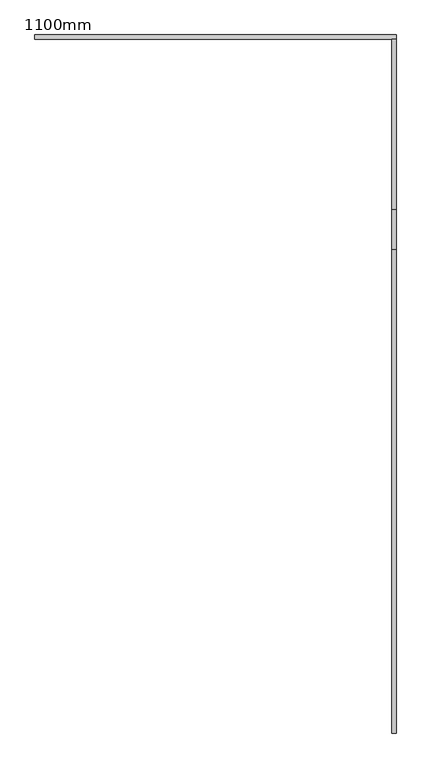
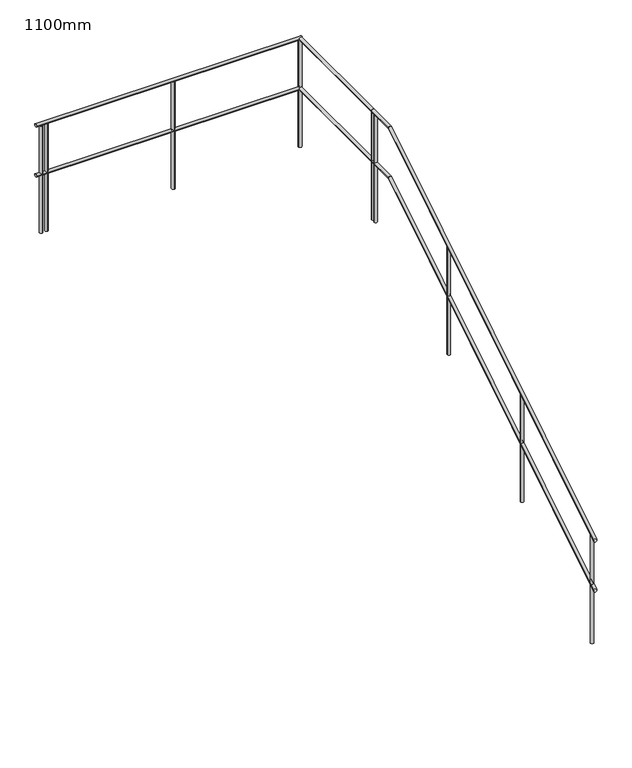
"""IFC4 building model written with IfcOpenShell, lengths in millimetres: railing geometry, 1100mm."""

from ifc_helpers import new_model, si_unit, point, frame, frame_2d, origin, place, context, project, spatial, circle_curve, ellipse_curve, trimmed, segment, composite_curve, outline, extrude, source, transform, mapped, element, save
from ifc_brep_helpers import plane_surface, cylinder_surface, advanced_brep


def railing_1100mm_b1036d3c(model_context):
    return source(origin(), model_context, "Body", "SolidModel", [
        advanced_brep(
        [(12740.5052251, 14699.5208589, 456.3396197), (12710.5052251, 14699.5208589, 456.3396197), (12740.5052251, 18339.5208589, 2547.0), (12710.5052251, 18339.5208589, 2547.0), (12740.5052251, 18063.8019306, 2547.0), (12710.5052251, 18063.8019306, 2547.0)],
        [
            (0, 1, ellipse_curve(frame((12725.5052251, 14699.5208589, 456.3396197), z_axis=(0.0, -1.0, 0.0), x_axis=(0.0, 0.0, -1.0)), 17.6603803, 15.0)),
            (1, 0, ellipse_curve(frame((12725.5052251, 14699.5208589, 456.3396197), z_axis=(0.0, -1.0, 0.0), x_axis=(0.0, 0.0, -1.0)), 17.6603803, 15.0)),
            (2, 3, circle_curve(frame((12725.5052251, 18339.5208589, 2547.0), z_axis=(0.0, 1.0, 0.0), x_axis=(-1.0, 0.0, 0.0)), 15.0)),
            (3, 2, circle_curve(frame((12725.5052251, 18339.5208589, 2547.0), z_axis=(0.0, 1.0, 0.0), x_axis=(-1.0, 0.0, 0.0)), 15.0)),
            (0, 4),
            (4, 5, ellipse_curve(frame((12725.5052251, 18063.8019306, 2547.0), z_axis=(0.0, -0.9616025257983003, -0.2744459552959912), x_axis=(0.0, 0.2744459552959914, -0.9616025257983002)), 15.5989607, 15.0)),
            (5, 1),
            (5, 4, ellipse_curve(frame((12725.5052251, 18063.8019306, 2547.0), z_axis=(0.0, -0.9616025257983003, -0.2744459552959912), x_axis=(0.0, 0.2744459552959914, -0.9616025257983002)), 15.5989607, 15.0)),
            (4, 2),
            (3, 5),
        ],
        [
            plane_surface(frame((12725.5052251, 14699.5208589, 474.0), z_axis=(0.0, -1.0, 0.0), x_axis=(0.0, 0.0, 1.0))),
            plane_surface(frame((12725.5052251, 18339.5208589, 2562.0), z_axis=(0.0, 1.0, 0.0), x_axis=(0.0, 0.0, 1.0))),
            cylinder_surface(frame((12725.5052251, 14707.4380966, 461.2596175), z_axis=(0.0, -0.8493588352433417, -0.5278158476155052), x_axis=(-1.0, 0.0, 0.0)), 15.0),
            cylinder_surface(frame((12725.5052251, 18059.5208589, 2547.0), z_axis=(0.0, -1.0, 0.0), x_axis=(-1.0, 0.0, 0.0)), 15.0),
        ],
        [
            (0, [[1, 2]]),
            (1, [[3, 4]]),
            (2, [[-1, 5, 6, 7]]),
            (2, [[-2, -7, 8, -5]]),
            (3, [[-6, 9, -4, 10]]),
            (3, [[-8, -10, -3, -9]]),
        ],
    ),
        advanced_brep(
        [(12740.5052251, 18339.5208589, 2547.0), (12710.5052251, 18339.5208589, 2547.0), (12740.5052251, 19524.9208589, 2547.0), (12710.5052251, 19524.9208589, 2547.0)],
        [
            (0, 1, circle_curve(frame((12725.5052251, 18339.5208589, 2547.0), z_axis=(0.0, -1.0, 0.0), x_axis=(-1.0, 0.0, 0.0)), 15.0)),
            (1, 0, circle_curve(frame((12725.5052251, 18339.5208589, 2547.0), z_axis=(0.0, -1.0, 0.0), x_axis=(-1.0, 0.0, 0.0)), 15.0)),
            (2, 3, circle_curve(frame((12725.5052251, 19524.9208589, 2547.0), z_axis=(0.0, 1.0, 0.0), x_axis=(-1.0, 0.0, 0.0)), 15.0)),
            (3, 2, circle_curve(frame((12725.5052251, 19524.9208589, 2547.0), z_axis=(0.0, 1.0, 0.0), x_axis=(-1.0, 0.0, 0.0)), 15.0)),
            (0, 2),
            (3, 1),
        ],
        [
            plane_surface(frame((12725.5052251, 18339.5208589, 2562.0), z_axis=(0.0, -1.0, 0.0), x_axis=(0.0, 0.0, 1.0))),
            plane_surface(frame((12725.5052251, 19524.9208589, 2562.0), z_axis=(0.0, 1.0, 0.0), x_axis=(0.0, 0.0, 1.0))),
            cylinder_surface(frame((12725.5052251, 18339.5208589, 2547.0), z_axis=(0.0, -1.0, 0.0), x_axis=(-1.0, 0.0, 0.0)), 15.0),
        ],
        [
            (0, [[1, 2]]),
            (1, [[3, 4]]),
            (2, [[-1, 5, -4, 6]]),
            (2, [[-2, -6, -3, -5]]),
        ],
    ),
        advanced_brep(
        [(12740.5052251, 19554.9208589, 2547.0), (12740.5052251, 19524.9208589, 2547.0), (10225.1052251, 19554.9208589, 2547.0), (10225.1052251, 19524.9208589, 2547.0)],
        [
            (0, 1, circle_curve(frame((12740.5052251, 19539.9208589, 2547.0), z_axis=(1.0, 0.0, 0.0), x_axis=(0.0, -1.0, 0.0)), 15.0)),
            (1, 0, circle_curve(frame((12740.5052251, 19539.9208589, 2547.0), z_axis=(1.0, 0.0, 0.0), x_axis=(0.0, -1.0, 0.0)), 15.0)),
            (2, 3, circle_curve(frame((10225.1052251, 19539.9208589, 2547.0), z_axis=(-1.0, 0.0, 0.0), x_axis=(0.0, -1.0, 0.0)), 15.0)),
            (3, 2, circle_curve(frame((10225.1052251, 19539.9208589, 2547.0), z_axis=(-1.0, 0.0, 0.0), x_axis=(0.0, -1.0, 0.0)), 15.0)),
            (0, 2),
            (3, 1),
        ],
        [
            plane_surface(frame((12740.5052251, 19539.9208589, 2562.0), z_axis=(1.0, 0.0, 0.0), x_axis=(0.0, -1.0, 0.0))),
            plane_surface(frame((10225.1052251, 19539.9208589, 2562.0), z_axis=(-1.0, 0.0, 0.0), x_axis=(0.0, -1.0, 0.0))),
            cylinder_surface(frame((12740.5052251, 19539.9208589, 2547.0), z_axis=(1.0, 0.0, 0.0), x_axis=(0.0, -1.0, 0.0)), 15.0),
        ],
        [
            (0, [[1, 2]]),
            (1, [[3, 4]]),
            (2, [[-1, 5, -4, 6]]),
            (2, [[-2, -6, -3, -5]]),
        ],
    ),
        advanced_brep(
        [(12740.5052251, 14699.5208589, 956.3396197), (12710.5052251, 14699.5208589, 956.3396197), (12740.5052251, 18063.8019306, 3047.0), (12710.5052251, 18063.8019306, 3047.0), (12740.5052251, 18339.5208589, 3047.0), (12710.5052251, 18339.5208589, 3047.0)],
        [
            (0, 1, ellipse_curve(frame((12725.5052251, 14699.5208589, 956.3396197), z_axis=(0.0, -1.0, 0.0), x_axis=(0.0, 0.0, -1.0)), 17.6603803, 15.0)),
            (1, 0, ellipse_curve(frame((12725.5052251, 14699.5208589, 956.3396197), z_axis=(0.0, -1.0, 0.0), x_axis=(0.0, 0.0, -1.0)), 17.6603803, 15.0)),
            (0, 2),
            (2, 3, ellipse_curve(frame((12725.5052251, 18063.8019306, 3047.0), z_axis=(0.0, -0.9616025257983003, -0.2744459552959912), x_axis=(0.0, 0.2744459552959914, -0.9616025257983002)), 15.5989607, 15.0)),
            (3, 1),
            (3, 2, ellipse_curve(frame((12725.5052251, 18063.8019306, 3047.0), z_axis=(0.0, -0.9616025257983003, -0.2744459552959912), x_axis=(0.0, 0.2744459552959914, -0.9616025257983002)), 15.5989607, 15.0)),
            (4, 5, circle_curve(frame((12725.5052251, 18339.5208589, 3047.0), z_axis=(0.0, 1.0, 0.0), x_axis=(-1.0, 0.0, 0.0)), 15.0)),
            (5, 4, circle_curve(frame((12725.5052251, 18339.5208589, 3047.0), z_axis=(0.0, 1.0, 0.0), x_axis=(-1.0, 0.0, 0.0)), 15.0)),
            (2, 4),
            (5, 3),
        ],
        [
            plane_surface(frame((12725.5052251, 14699.5208589, 974.0), z_axis=(0.0, -1.0, 0.0), x_axis=(0.0, 0.0, 1.0))),
            cylinder_surface(frame((12725.5052251, 14707.4380966, 961.2596175), z_axis=(0.0, -0.8493588352433417, -0.5278158476155052), x_axis=(-1.0, 0.0, 0.0)), 15.0),
            plane_surface(frame((12725.5052251, 18339.5208589, 3062.0), z_axis=(0.0, 1.0, 0.0), x_axis=(0.0, 0.0, 1.0))),
            cylinder_surface(frame((12725.5052251, 18059.5208589, 3047.0), z_axis=(0.0, -1.0, 0.0), x_axis=(-1.0, 0.0, 0.0)), 15.0),
        ],
        [
            (0, [[1, 2]]),
            (1, [[-1, 3, 4, 5]]),
            (1, [[-2, -5, 6, -3]]),
            (2, [[7, 8]]),
            (3, [[-4, 9, -8, 10]]),
            (3, [[-6, -10, -7, -9]]),
        ],
    ),
        advanced_brep(
        [(12740.5052251, 18339.5208589, 3047.0), (12710.5052251, 18339.5208589, 3047.0), (12740.5052251, 19524.9208589, 3047.0), (12710.5052251, 19524.9208589, 3047.0)],
        [
            (0, 1, circle_curve(frame((12725.5052251, 18339.5208589, 3047.0), z_axis=(0.0, -1.0, 0.0), x_axis=(-1.0, 0.0, 0.0)), 15.0)),
            (1, 0, circle_curve(frame((12725.5052251, 18339.5208589, 3047.0), z_axis=(0.0, -1.0, 0.0), x_axis=(-1.0, 0.0, 0.0)), 15.0)),
            (2, 3, circle_curve(frame((12725.5052251, 19524.9208589, 3047.0), z_axis=(0.0, 1.0, 0.0), x_axis=(-1.0, 0.0, 0.0)), 15.0)),
            (3, 2, circle_curve(frame((12725.5052251, 19524.9208589, 3047.0), z_axis=(0.0, 1.0, 0.0), x_axis=(-1.0, 0.0, 0.0)), 15.0)),
            (0, 2),
            (3, 1),
        ],
        [
            plane_surface(frame((12725.5052251, 18339.5208589, 3062.0), z_axis=(0.0, -1.0, 0.0), x_axis=(0.0, 0.0, 1.0))),
            plane_surface(frame((12725.5052251, 19524.9208589, 3062.0), z_axis=(0.0, 1.0, 0.0), x_axis=(0.0, 0.0, 1.0))),
            cylinder_surface(frame((12725.5052251, 18339.5208589, 3047.0), z_axis=(0.0, -1.0, 0.0), x_axis=(-1.0, 0.0, 0.0)), 15.0),
        ],
        [
            (0, [[1, 2]]),
            (1, [[3, 4]]),
            (2, [[-1, 5, -4, 6]]),
            (2, [[-2, -6, -3, -5]]),
        ],
    ),
        advanced_brep(
        [(12740.5052251, 19554.9208589, 3047.0), (12740.5052251, 19524.9208589, 3047.0), (10225.1052251, 19554.9208589, 3047.0), (10225.1052251, 19524.9208589, 3047.0)],
        [
            (0, 1, circle_curve(frame((12740.5052251, 19539.9208589, 3047.0), z_axis=(1.0, 0.0, 0.0), x_axis=(0.0, -1.0, 0.0)), 15.0)),
            (1, 0, circle_curve(frame((12740.5052251, 19539.9208589, 3047.0), z_axis=(1.0, 0.0, 0.0), x_axis=(0.0, -1.0, 0.0)), 15.0)),
            (2, 3, circle_curve(frame((10225.1052251, 19539.9208589, 3047.0), z_axis=(-1.0, 0.0, 0.0), x_axis=(0.0, -1.0, 0.0)), 15.0)),
            (3, 2, circle_curve(frame((10225.1052251, 19539.9208589, 3047.0), z_axis=(-1.0, 0.0, 0.0), x_axis=(0.0, -1.0, 0.0)), 15.0)),
            (0, 2),
            (3, 1),
        ],
        [
            plane_surface(frame((12740.5052251, 19539.9208589, 3062.0), z_axis=(1.0, 0.0, 0.0), x_axis=(0.0, -1.0, 0.0))),
            plane_surface(frame((10225.1052251, 19539.9208589, 3062.0), z_axis=(-1.0, 0.0, 0.0), x_axis=(0.0, -1.0, 0.0))),
            cylinder_surface(frame((12740.5052251, 19539.9208589, 3047.0), z_axis=(1.0, 0.0, 0.0), x_axis=(0.0, -1.0, 0.0)), 15.0),
        ],
        [
            (0, [[1, 2]]),
            (1, [[3, 4]]),
            (2, [[-1, 5, -4, 6]]),
            (2, [[-2, -6, -3, -5]]),
        ],
    ),
        extrude(outline(composite_curve([segment(trimmed(circle_curve(frame_2d((10325.5052251, 19539.9208589)), 15.0), [point((10325.5052251, 19524.9208589))], [point((10325.5052251, 19554.9208589))], False, "CARTESIAN"), True, "CONTINUOUS"), segment(trimmed(circle_curve(frame_2d((10325.5052251, 19539.9208589)), 15.0), [point((10325.5052251, 19554.9208589))], [point((10325.5052251, 19524.9208589))], False, "CARTESIAN"), True, "CONTINUOUS")], self_intersect=False)), frame((0.0, 0.0, 1962.0), z_axis=(0.0, 0.0, 1.0), x_axis=(1.0, 0.0, 0.0)), (0.0, 0.0, 1.0), 1070.0),
        extrude(outline(composite_curve([segment(trimmed(circle_curve(frame_2d((11525.5052251, 19539.9208589)), 15.0), [point((11525.5052251, 19524.9208589))], [point((11525.5052251, 19554.9208589))], False, "CARTESIAN"), True, "CONTINUOUS"), segment(trimmed(circle_curve(frame_2d((11525.5052251, 19539.9208589)), 15.0), [point((11525.5052251, 19554.9208589))], [point((11525.5052251, 19524.9208589))], False, "CARTESIAN"), True, "CONTINUOUS")], self_intersect=False)), frame((0.0, 0.0, 1962.0), z_axis=(0.0, 0.0, 1.0), x_axis=(1.0, 0.0, 0.0)), (0.0, 0.0, 1.0), 1070.0),
        extrude(outline(composite_curve([segment(trimmed(circle_curve(frame_2d((12725.5052251, 19539.5208589)), 15.0), [point((12710.5052251, 19539.5208589))], [point((12740.5052251, 19539.5208589))], False, "CARTESIAN"), True, "CONTINUOUS"), segment(trimmed(circle_curve(frame_2d((12725.5052251, 19539.5208589)), 15.0), [point((12740.5052251, 19539.5208589))], [point((12710.5052251, 19539.5208589))], False, "CARTESIAN"), True, "CONTINUOUS")], self_intersect=False)), frame((0.0, 0.0, 1962.0), z_axis=(0.0, 0.0, 1.0), x_axis=(1.0, 0.0, 0.0)), (0.0, 0.0, 1.0), 1070.0),
        extrude(outline(composite_curve([segment(trimmed(circle_curve(frame_2d((12725.5052251, 18299.5208589)), 15.0), [point((12710.5052251, 18299.5208589))], [point((12740.5052251, 18299.5208589))], False, "CARTESIAN"), True, "CONTINUOUS"), segment(trimmed(circle_curve(frame_2d((12725.5052251, 18299.5208589)), 15.0), [point((12740.5052251, 18299.5208589))], [point((12710.5052251, 18299.5208589))], False, "CARTESIAN"), True, "CONTINUOUS")], self_intersect=False)), frame((0.0, 0.0, 1962.0), z_axis=(0.0, 0.0, 1.0), x_axis=(1.0, 0.0, 0.0)), (0.0, 0.0, 1.0), 1070.0),
        extrude(outline(composite_curve([segment(trimmed(circle_curve(frame_2d((12725.5052251, 17099.5208589)), 15.0), [point((12710.5052251, 17099.5208589))], [point((12740.5052251, 17099.5208589))], False, "CARTESIAN"), True, "CONTINUOUS"), segment(trimmed(circle_curve(frame_2d((12725.5052251, 17099.5208589)), 15.0), [point((12740.5052251, 17099.5208589))], [point((12710.5052251, 17099.5208589))], False, "CARTESIAN"), True, "CONTINUOUS")], self_intersect=False)), frame((0.0, 0.0, 1365.4285714), z_axis=(0.0, 0.0, 1.0), x_axis=(1.0, 0.0, 0.0)), (0.0, 0.0, 1.0), 1070.0),
        extrude(outline(composite_curve([segment(trimmed(circle_curve(frame_2d((12725.5052251, 15899.5208589)), 15.0), [point((12710.5052251, 15899.5208589))], [point((12740.5052251, 15899.5208589))], False, "CARTESIAN"), True, "CONTINUOUS"), segment(trimmed(circle_curve(frame_2d((12725.5052251, 15899.5208589)), 15.0), [point((12740.5052251, 15899.5208589))], [point((12710.5052251, 15899.5208589))], False, "CARTESIAN"), True, "CONTINUOUS")], self_intersect=False)), frame((0.0, 0.0, 619.7142857), z_axis=(0.0, 0.0, 1.0), x_axis=(1.0, 0.0, 0.0)), (0.0, 0.0, 1.0), 1070.0),
        extrude(outline(composite_curve([segment(trimmed(circle_curve(frame_2d((12725.5052251, 19539.9208589)), 15.0), [point((12710.5052251, 19539.9208589))], [point((12740.5052251, 19539.9208589))], False, "CARTESIAN"), True, "CONTINUOUS"), segment(trimmed(circle_curve(frame_2d((12725.5052251, 19539.9208589)), 15.0), [point((12740.5052251, 19539.9208589))], [point((12710.5052251, 19539.9208589))], False, "CARTESIAN"), True, "CONTINUOUS")], self_intersect=False)), frame((0.0, 0.0, 1962.0), z_axis=(0.0, 0.0, 1.0), x_axis=(1.0, 0.0, 0.0)), (0.0, 0.0, 1.0), 1070.0),
        extrude(outline(composite_curve([segment(trimmed(circle_curve(frame_2d((12725.5052251, 18339.5208589)), 15.0), [point((12710.5052251, 18339.5208589))], [point((12740.5052251, 18339.5208589))], False, "CARTESIAN"), True, "CONTINUOUS"), segment(trimmed(circle_curve(frame_2d((12725.5052251, 18339.5208589)), 15.0), [point((12740.5052251, 18339.5208589))], [point((12710.5052251, 18339.5208589))], False, "CARTESIAN"), True, "CONTINUOUS")], self_intersect=False)), frame((0.0, 0.0, 1962.0), z_axis=(0.0, 0.0, 1.0), x_axis=(1.0, 0.0, 0.0)), (0.0, 0.0, 1.0), 1070.0),
        extrude(outline(composite_curve([segment(trimmed(circle_curve(frame_2d((10275.1052251, 19539.9208589)), 15.0), [point((10275.1052251, 19524.9208589))], [point((10275.1052251, 19554.9208589))], False, "CARTESIAN"), True, "CONTINUOUS"), segment(trimmed(circle_curve(frame_2d((10275.1052251, 19539.9208589)), 15.0), [point((10275.1052251, 19554.9208589))], [point((10275.1052251, 19524.9208589))], False, "CARTESIAN"), True, "CONTINUOUS")], self_intersect=False)), frame((0.0, 0.0, 1962.0), z_axis=(0.0, 0.0, 1.0), x_axis=(1.0, 0.0, 0.0)), (0.0, 0.0, 1.0), 1070.0),
        extrude(outline(composite_curve([segment(trimmed(circle_curve(frame_2d((12725.5052251, 14749.5208589)), 15.0), [point((12710.5052251, 14749.5208589))], [point((12740.5052251, 14749.5208589))], False, "CARTESIAN"), True, "CONTINUOUS"), segment(trimmed(circle_curve(frame_2d((12725.5052251, 14749.5208589)), 15.0), [point((12740.5052251, 14749.5208589))], [point((12710.5052251, 14749.5208589))], False, "CARTESIAN"), True, "CONTINUOUS")], self_intersect=False)), frame((0.0, 0.0, -94.9285714), z_axis=(0.0, 0.0, 1.0), x_axis=(1.0, 0.0, 0.0)), (0.0, 0.0, 1.0), 1070.0),
    ])


if __name__ == "__main__":
    model = new_model("IFC4")
    model_context = context("Model", 3, world=origin())
    ifc_project = project(units=[si_unit("LENGTHUNIT", "METRE", prefix="MILLI")], contexts=[model_context])
    site = spatial("IfcSite", under=ifc_project)
    building = spatial("IfcBuilding", under=site)
    placement = place(None, origin())
    railing_1100mm_shape = railing_1100mm_b1036d3c(model_context)
    element("IfcRailing", 1, ObjectType="1100mm", at=placement, inside=building, context=model_context, shape_type="MappedRepresentation", body=[
        mapped(railing_1100mm_shape, transform((0.0, 0.0, 0.0), x_axis=(1.0, 0.0, 0.0), y_axis=(0.0, 1.0, 0.0), z_axis=(0.0, 0.0, 1.0))),
    ])
    save(model, "model.ifc")
